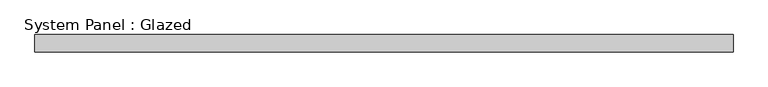
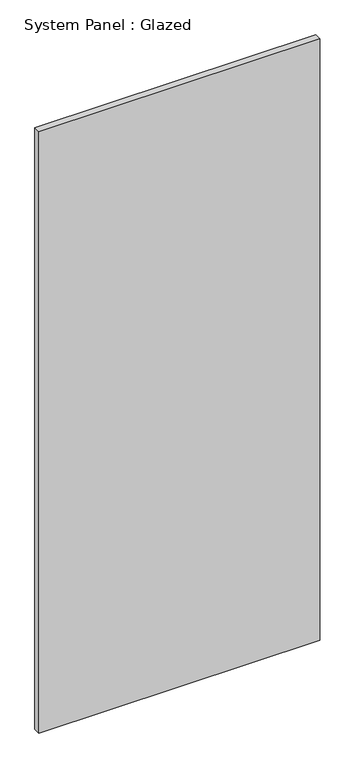
"""IFC4 building model written with IfcOpenShell, lengths in millimetres: plate geometry, System Panel : Glazed."""

import ifcopenshell
import ifcopenshell.guid

model = None  # the IFC model being written
_history = None  # IfcOwnerHistory: only IFC2X3 demands one
_inside = {}  # id of a spatial element -> (the spatial element, [elements in it])
_under = {}  # id of a project, library or spatial element -> (it, [spatial elements below it])
_declared = {}  # id of a project -> (the project, [libraries it declares])
_typed = {}  # id of a type object -> (the type object, [elements of that type])
_made_of = {}  # id of a material, layer set ... -> (it, [elements and type objects made of it])


def new_model(schema):
    """Start an empty IFC model of exactly this schema.

    Asked for "IFC4X3", IfcOpenShell would pick the latest addendum, in which some entities
    have other attributes; the version numbers below select the first issue.
    IFC2X3 requires an IfcOwnerHistory on every rooted entity: one is made here for all.
    """
    global model, _history
    if schema == "IFC4X3":
        model = ifcopenshell.file(schema_version=(4, 3, 0, 0))
    else:
        model = ifcopenshell.file(schema=schema)
    _inside.clear()
    _under.clear()
    _declared.clear()
    _typed.clear()
    _made_of.clear()
    _history = None
    if model.schema == "IFC2X3":
        org = make("IfcOrganization", Name="unknown")
        user = make(
            "IfcPersonAndOrganization",
            ThePerson=make("IfcPerson", FamilyName="unknown"),
            TheOrganization=org,
        )
        app = make(
            "IfcApplication",
            ApplicationDeveloper=org,
            Version="unknown",
            ApplicationFullName="unknown",
            ApplicationIdentifier="unknown",
        )
        _history = make(
            "IfcOwnerHistory",
            OwningUser=user,
            OwningApplication=app,
            ChangeAction="ADDED",
            CreationDate=0,
        )
    return model


def make(cls, **values):
    """One entity of the class cls with the attributes given. An attribute that is None is left unset."""
    return model.create_entity(
        cls, **{name: value for name, value in values.items() if value is not None}
    )


def rooted(cls, **values):
    """An entity with a GlobalId (a new one), such as an element, a storey or a relation."""
    return make(cls, GlobalId=ifcopenshell.guid.new(), OwnerHistory=_history, **values)


def si_unit(unit_type, name, prefix=None):
    """IfcSIUnit, for example si_unit("LENGTHUNIT", "METRE", prefix="MILLI")."""
    return make("IfcSIUnit", UnitType=unit_type, Prefix=prefix, Name=name)


def assignment(units):
    """IfcUnitAssignment: the units of a project."""
    return None if units is None else make("IfcUnitAssignment", Units=units)


def point(xyz):
    """IfcCartesianPoint."""
    return None if xyz is None else make("IfcCartesianPoint", Coordinates=xyz)


def direction(xyz):
    """IfcDirection."""
    return None if xyz is None else make("IfcDirection", DirectionRatios=xyz)


def frame(location, z_axis=None, x_axis=None):
    """IfcAxis2Placement3D, a coordinate frame: its origin and axes. An axis left out is left unset."""
    return make(
        "IfcAxis2Placement3D",
        Location=point(location),
        Axis=direction(z_axis),
        RefDirection=direction(x_axis),
    )


def origin():
    """The frame at (0, 0, 0) with its axes left unset."""
    return frame((0.0, 0.0, 0.0))


def origin_with_axes():
    """The frame at (0, 0, 0) with the z axis (0, 0, 1) and the x axis (1, 0, 0) written out."""
    return frame((0.0, 0.0, 0.0), z_axis=(0.0, 0.0, 1.0), x_axis=(1.0, 0.0, 0.0))


def place(relative_to, where):
    """IfcLocalPlacement: puts the frame where relative to a parent placement (None: the world)."""
    return make(
        "IfcLocalPlacement", PlacementRelTo=relative_to, RelativePlacement=where
    )


def context(
    kind, dimensions, precision=None, world=None, true_north=None, identifier=None
):
    """IfcGeometricRepresentationContext, for example the 3D "Model" context."""
    return make(
        "IfcGeometricRepresentationContext",
        ContextIdentifier=identifier,
        ContextType=kind,
        CoordinateSpaceDimension=dimensions,
        Precision=precision,
        WorldCoordinateSystem=world,
        TrueNorth=true_north,
    )


def project(units=None, contexts=None):
    """IfcProject with its units and contexts."""
    return rooted(
        "IfcProject",
        Name="project",
        RepresentationContexts=contexts,
        UnitsInContext=assignment(units),
    )


def spatial(cls, under=None, at=None, **own):
    """A site, building, storey or space (cls), placed at a placement, below another one or the project."""
    s = rooted(cls, ObjectPlacement=at, **own)
    if under is not None:
        _under.setdefault(under.id(), (under, []))[1].append(s)
    return s


def polyline(points):
    """IfcPolyline through the points."""
    return make("IfcPolyline", Points=[point(p) for p in points])


def outline(outer, holes=None, kind="AREA"):
    """IfcArbitraryClosedProfileDef: a profile drawn as a closed curve; with holes, ...WithVoids."""
    if holes is None:
        return make("IfcArbitraryClosedProfileDef", ProfileType=kind, OuterCurve=outer)
    return make(
        "IfcArbitraryProfileDefWithVoids",
        ProfileType=kind,
        OuterCurve=outer,
        InnerCurves=holes,
    )


def extrude(swept, where, along, depth):
    """IfcExtrudedAreaSolid: the profile swept, set in the frame where, extruded along a direction by depth."""
    return make(
        "IfcExtrudedAreaSolid",
        SweptArea=swept,
        Position=where,
        ExtrudedDirection=direction(along),
        Depth=depth,
    )


def shape(context_of_items, identifier, shape_type, items):
    """IfcShapeRepresentation: the items that make up one representation, for example the "Body"."""
    return make(
        "IfcShapeRepresentation",
        ContextOfItems=context_of_items,
        RepresentationIdentifier=identifier,
        RepresentationType=shape_type,
        Items=items,
    )


def source(mapping_origin, context_of_items, identifier, shape_type, items):
    """IfcRepresentationMap: a shape defined once, which mapped items show again and again."""
    return make(
        "IfcRepresentationMap",
        MappingOrigin=mapping_origin,
        MappedRepresentation=shape(context_of_items, identifier, shape_type, items),
    )


def transform(
    local_origin,
    x_axis=None,
    y_axis=None,
    z_axis=None,
    scale=None,
    scale2=None,
    scale3=None,
    uniform=True,
):
    """IfcCartesianTransformationOperator3D, or its non-uniform kind. x_axis, y_axis, z_axis: its Axis1, 2, 3."""
    if uniform:
        return make(
            "IfcCartesianTransformationOperator3D",
            Axis1=direction(x_axis),
            Axis2=direction(y_axis),
            LocalOrigin=point(local_origin),
            Scale=scale,
            Axis3=direction(z_axis),
        )
    return make(
        "IfcCartesianTransformationOperator3DnonUniform",
        Axis1=direction(x_axis),
        Axis2=direction(y_axis),
        LocalOrigin=point(local_origin),
        Scale=scale,
        Axis3=direction(z_axis),
        Scale2=scale2,
        Scale3=scale3,
    )


def mapped(mapping_source, mapping_target):
    """IfcMappedItem: shows the shape of a source again, moved by a transform."""
    return make(
        "IfcMappedItem", MappingSource=mapping_source, MappingTarget=mapping_target
    )


def made_of(thing, what):
    """Note that an element or type object is made of a material, layer set ...; save() writes the relation."""
    if what is not None:
        _made_of.setdefault(what.id(), (what, []))[1].append(thing)
    return thing


def element(
    cls,
    number,
    at=None,
    inside=None,
    cuts=None,
    type_object=None,
    material=None,
    context=None,
    identifier="Body",
    shape_type=None,
    held_by="IfcProductDefinitionShape",
    body=None,
    shapes=None,
    **own,
):
    """One element of the class cls, such as IfcWall. Its Tag is "e" and its number.

    at: its placement. inside: the storey or other place that contains it. cuts: it is an
    opening in that element (IfcRelVoidsElement). A single representation is given by context,
    identifier, shape_type and body (its items); several are given by shapes. held_by: the class
    of the entity that holds the representations. save() writes the other relations.
    """
    e = rooted(cls, Tag="e%d" % number, ObjectPlacement=at, **own)
    if body is not None:
        shapes = [shape(context, identifier, shape_type, body)]
    if shapes is not None:
        e.Representation = make(held_by, Representations=shapes)
    if inside is not None:
        _inside.setdefault(inside.id(), (inside, []))[1].append(e)
    if cuts is not None:
        rooted(
            "IfcRelVoidsElement", RelatingBuildingElement=cuts, RelatedOpeningElement=e
        )
    if type_object is not None:
        _typed.setdefault(type_object.id(), (type_object, []))[1].append(e)
    return made_of(e, material)


def aggregate(whole, parts):
    """IfcRelAggregates: a whole, such as a stair, and the parts it consists of."""
    return rooted("IfcRelAggregates", RelatingObject=whole, RelatedObjects=parts)


def save(model, path):
    """Write the relations noted so far, then the file.

    IfcRelAggregates (storeys below a building ...), IfcRelContainedInSpatialStructure (elements
    in a storey), IfcRelDefinesByType, IfcRelAssociatesMaterial and IfcRelDeclares: one each for
    every whole, place, type object, material and project.
    """
    for whole, parts in _under.values():
        aggregate(whole, parts)
    for where, things in _inside.values():
        rooted(
            "IfcRelContainedInSpatialStructure",
            RelatedElements=things,
            RelatingStructure=where,
        )
    for kind, things in _typed.values():
        rooted("IfcRelDefinesByType", RelatedObjects=things, RelatingType=kind)
    for what, things in _made_of.values():
        rooted("IfcRelAssociatesMaterial", RelatedObjects=things, RelatingMaterial=what)
    for by, libraries in _declared.values():
        rooted("IfcRelDeclares", RelatingContext=by, RelatedDefinitions=libraries)
    model.write(path)


def system_panel_glazed_e676b032(model_context):
    return source(origin(), model_context, "Body", "SweptSolid", [
        extrude(outline(polyline([(517.525, 19.05), (-517.525, 19.05), (-517.525, 44.45), (517.525, 44.45), (517.525, 19.05)])), origin_with_axes(), (0.0, 0.0, 1.0), 2343.15),
    ])


if __name__ == "__main__":
    model = new_model("IFC4")
    model_context = context("Model", 3, world=origin())
    ifc_project = project(units=[si_unit("LENGTHUNIT", "METRE", prefix="MILLI")], contexts=[model_context])
    site = spatial("IfcSite", under=ifc_project)
    building = spatial("IfcBuilding", under=site)
    placement = place(None, origin())
    system_panel_glazed_shape = system_panel_glazed_e676b032(model_context)
    element("IfcPlate", 1, ObjectType="System Panel : Glazed", at=placement, inside=building, context=model_context, shape_type="MappedRepresentation", body=[
        mapped(system_panel_glazed_shape, transform((0.0, 0.0, 0.0), x_axis=(1.0, 0.0, 0.0), y_axis=(0.0, 1.0, 0.0), z_axis=(0.0, 0.0, 1.0))),
    ])
    save(model, "model.ifc")

# Revit data of these elements
# Element 1 (IfcPlate, "System Panel : Glazed")
#   Materials on its faces: "Glass"
# Materials
#   "Glass": class "Glass", colour RGB 0 128 192, transparency 0.75
